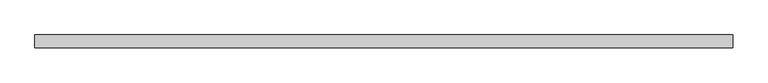
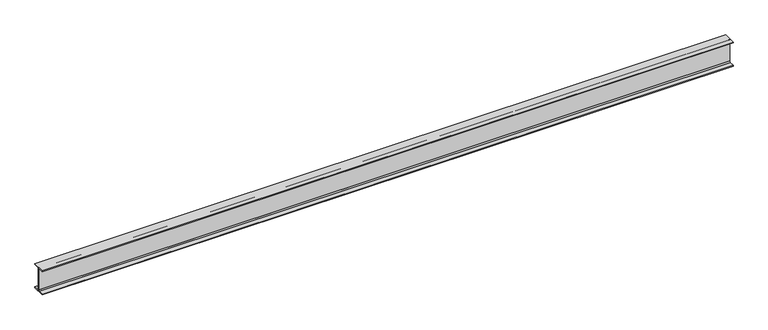
"""IFC4 building model written with IfcOpenShell, lengths in millimetres: beam geometry, 0912_Steel Framing_H-KSD3502 : H_SB_ASB_H-350x175x7x11."""

from ifc_helpers import new_model, si_unit, point, frame, frame_2d, origin, place, context, project, spatial, polyline, circle_curve, trimmed, segment, composite_curve, outline, extrude, source, transform, mapped, element, save


def beam_f28858a7(model_context):
    return source(origin(), model_context, "Body", "SweptSolid", [
        extrude(outline(composite_curve([segment(polyline([(87.5, -164.0), (87.5, -175.0), (-87.5, -175.0), (-87.5, -164.0), (-17.5, -164.0)]), True, "CONTINUOUS"), segment(trimmed(circle_curve(frame_2d((-17.5, -150.0)), 14.0), [point((-17.5, -164.0))], [point((-3.5, -150.0))], True, "CARTESIAN"), True, "CONTINUOUS"), segment(polyline([(-3.5, -150.0), (-3.5, 150.0)]), True, "CONTINUOUS"), segment(trimmed(circle_curve(frame_2d((-17.5, 150.0)), 14.0), [point((-3.5, 150.0))], [point((-17.5, 164.0))], True, "CARTESIAN"), True, "CONTINUOUS"), segment(polyline([(-17.5, 164.0), (-87.5, 164.0), (-87.5, 175.0), (87.5, 175.0), (87.5, 164.0), (17.5, 164.0)]), True, "CONTINUOUS"), segment(trimmed(circle_curve(frame_2d((17.5, 150.0)), 14.0), [point((17.5, 164.0))], [point((3.5, 150.0))], True, "CARTESIAN"), True, "CONTINUOUS"), segment(polyline([(3.5, 150.0), (3.5, -150.0)]), True, "CONTINUOUS"), segment(trimmed(circle_curve(frame_2d((17.5, -150.0)), 14.0), [point((3.5, -150.0))], [point((17.5, -164.0))], True, "CARTESIAN"), True, "CONTINUOUS"), segment(polyline([(17.5, -164.0), (87.5, -164.0)]), True, "CONTINUOUS")], self_intersect=False)), frame((-4664.4729123, 0.0, 0.0), z_axis=(1.0, 0.0, 0.0), x_axis=(0.0, 1.0, 0.0)), (0.0, 0.0, 1.0), 9526.7729123),
    ])


if __name__ == "__main__":
    model = new_model("IFC4")
    model_context = context("Model", 3, world=origin())
    ifc_project = project(units=[si_unit("LENGTHUNIT", "METRE", prefix="MILLI")], contexts=[model_context])
    site = spatial("IfcSite", under=ifc_project)
    building = spatial("IfcBuilding", under=site)
    placement = place(None, origin())
    beam_shape = beam_f28858a7(model_context)
    element("IfcBeam", 1, ObjectType="0912_Steel Framing_H-KSD3502 : H_SB_ASB_H-350x175x7x11", at=placement, inside=building, context=model_context, shape_type="MappedRepresentation", body=[
        mapped(beam_shape, transform((0.0, 0.0, 0.0), x_axis=(1.0, 0.0, 0.0), y_axis=(0.0, 1.0, 0.0), z_axis=(0.0, 0.0, 1.0))),
    ])
    save(model, "model.ifc")

# Revit data of these elements
# Type "0912_Steel Framing_H-KSD3502 : H_SB_ASB_H-350x175x7x11"
#   H_WM Code_1 = "S01AA002-00001 | Main Steel Structure Fabrication Work | Shelter/Building | Medium Steel - Standard (90KG/M>Weight≥30KG/M) | Material: (   )"
#   H_WM Code_2 = "S03AA028-00001 | Main Steel Structure Erection Work | Shelter/Building | Medium Steel (90KG/M>Weight≥30KG/M) | Material: (   )"
#   H_WM Code_3 = "S01AA010-00001 | Main Steel Structure Fabrication Work | Shelter/Building | Steel Painting/Coating | for Non-Fireproofed Steel Surface, Surface Preparation, Primer, Second & Final Coat | Material: (   )"
#   H_Q'ty Cal Type Tag = "SB-Q2"
#   Width = 17.5 cm
#   Web Thickness = 0.7 cm
#   Web Fillet = 1.4 cm
#   Warping Constant = 282000.0 cm⁶
#   W = 0
#   Torsional Moment of Inertia = 19.4042 cm⁴
#   Section Area = 63.14 cm²
#   Plastic Modulus weak axis = 174.0 cm³
#   Plastic Modulus strong axis = 868.0 cm³
#   Perimeter = 1.36 m²/m
#   Nominal Weight = 49.60 kgf/m
#   Moment of Inertia weak axis = 984.00 cm⁴
#   Moment of Inertia strong axis = 13600.00 cm⁴
#   Height = 35.0 cm
#   Flange Thickness = 1.1 cm
#   Elastic Modulus weak axis = 112.0 cm³
#   Elastic Modulus strong axis = 775.0 cm³
#   Centroid Vertical = 17.5 cm
#   Centroid Horizontal = 8.75 cm
#   Ix = 136000000
#   Length [instance default] = 1.5240 m
#   Zx = 868000
#   b = 0.1750 m
#   h = 0.3500 m
#   r = 0.0140 m
#   s = 0.0070 m
#   t = 0.0110 m
#   A = 0.006314 m²
#   Structural Material [instance default] = Steel, 45-345
#   Assembly Code = ""
# Element 1 (IfcBeam, "0912_Steel Framing_H-KSD3502 : H_SB_ASB_H-350x175x7x11")
#   Structural Material = none
# Materials
#   "Steel, 45-345": class "Metal", colour RGB 189 187 185, transparency 0, Description = "Steel 345 MPa", Cost = 0
